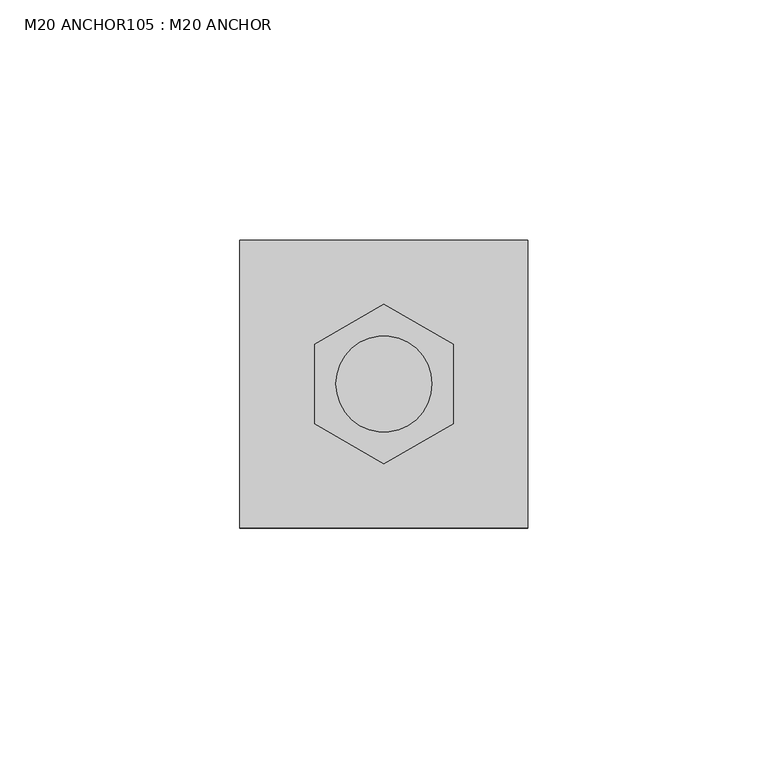
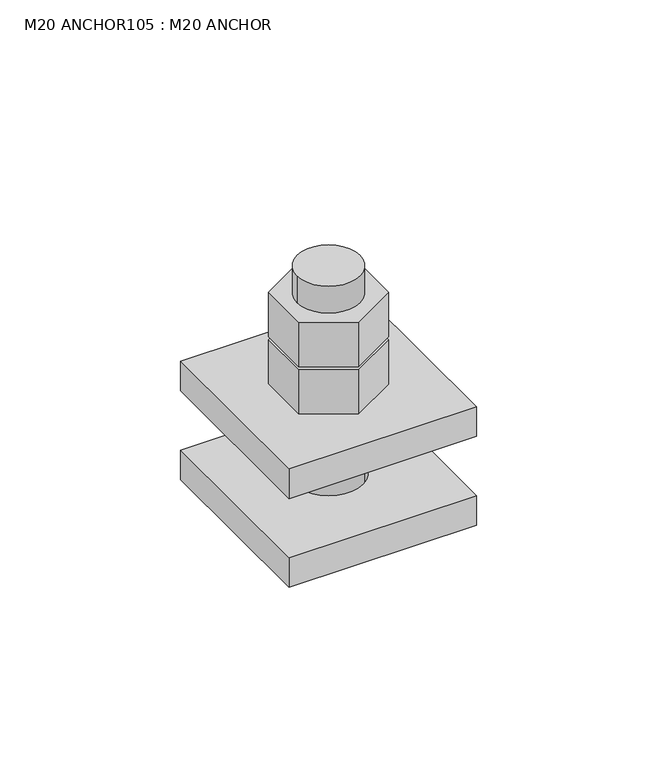
"""IFC4 building model written with IfcOpenShell, lengths in millimetres: fastener geometry, M20 ANCHOR105 : M20 ANCHOR."""

import ifcopenshell
import ifcopenshell.guid

model = None  # the IFC model being written
_history = None  # IfcOwnerHistory: only IFC2X3 demands one
_inside = {}  # id of a spatial element -> (the spatial element, [elements in it])
_under = {}  # id of a project, library or spatial element -> (it, [spatial elements below it])
_declared = {}  # id of a project -> (the project, [libraries it declares])
_typed = {}  # id of a type object -> (the type object, [elements of that type])
_made_of = {}  # id of a material, layer set ... -> (it, [elements and type objects made of it])


def new_model(schema):
    """Start an empty IFC model of exactly this schema.

    Asked for "IFC4X3", IfcOpenShell would pick the latest addendum, in which some entities
    have other attributes; the version numbers below select the first issue.
    IFC2X3 requires an IfcOwnerHistory on every rooted entity: one is made here for all.
    """
    global model, _history
    if schema == "IFC4X3":
        model = ifcopenshell.file(schema_version=(4, 3, 0, 0))
    else:
        model = ifcopenshell.file(schema=schema)
    _inside.clear()
    _under.clear()
    _declared.clear()
    _typed.clear()
    _made_of.clear()
    _history = None
    if model.schema == "IFC2X3":
        org = make("IfcOrganization", Name="unknown")
        user = make(
            "IfcPersonAndOrganization",
            ThePerson=make("IfcPerson", FamilyName="unknown"),
            TheOrganization=org,
        )
        app = make(
            "IfcApplication",
            ApplicationDeveloper=org,
            Version="unknown",
            ApplicationFullName="unknown",
            ApplicationIdentifier="unknown",
        )
        _history = make(
            "IfcOwnerHistory",
            OwningUser=user,
            OwningApplication=app,
            ChangeAction="ADDED",
            CreationDate=0,
        )
    return model


def make(cls, **values):
    """One entity of the class cls with the attributes given. An attribute that is None is left unset."""
    return model.create_entity(
        cls, **{name: value for name, value in values.items() if value is not None}
    )


def rooted(cls, **values):
    """An entity with a GlobalId (a new one), such as an element, a storey or a relation."""
    return make(cls, GlobalId=ifcopenshell.guid.new(), OwnerHistory=_history, **values)


def si_unit(unit_type, name, prefix=None):
    """IfcSIUnit, for example si_unit("LENGTHUNIT", "METRE", prefix="MILLI")."""
    return make("IfcSIUnit", UnitType=unit_type, Prefix=prefix, Name=name)


def assignment(units):
    """IfcUnitAssignment: the units of a project."""
    return None if units is None else make("IfcUnitAssignment", Units=units)


def point(xyz):
    """IfcCartesianPoint."""
    return None if xyz is None else make("IfcCartesianPoint", Coordinates=xyz)


def direction(xyz):
    """IfcDirection."""
    return None if xyz is None else make("IfcDirection", DirectionRatios=xyz)


def frame(location, z_axis=None, x_axis=None):
    """IfcAxis2Placement3D, a coordinate frame: its origin and axes. An axis left out is left unset."""
    return make(
        "IfcAxis2Placement3D",
        Location=point(location),
        Axis=direction(z_axis),
        RefDirection=direction(x_axis),
    )


def frame_2d(location, x_axis=None):
    """IfcAxis2Placement2D, a coordinate frame in the plane: its origin and x axis."""
    return make(
        "IfcAxis2Placement2D", Location=point(location), RefDirection=direction(x_axis)
    )


def origin():
    """The frame at (0, 0, 0) with its axes left unset."""
    return frame((0.0, 0.0, 0.0))


def place(relative_to, where):
    """IfcLocalPlacement: puts the frame where relative to a parent placement (None: the world)."""
    return make(
        "IfcLocalPlacement", PlacementRelTo=relative_to, RelativePlacement=where
    )


def context(
    kind, dimensions, precision=None, world=None, true_north=None, identifier=None
):
    """IfcGeometricRepresentationContext, for example the 3D "Model" context."""
    return make(
        "IfcGeometricRepresentationContext",
        ContextIdentifier=identifier,
        ContextType=kind,
        CoordinateSpaceDimension=dimensions,
        Precision=precision,
        WorldCoordinateSystem=world,
        TrueNorth=true_north,
    )


def project(units=None, contexts=None):
    """IfcProject with its units and contexts."""
    return rooted(
        "IfcProject",
        Name="project",
        RepresentationContexts=contexts,
        UnitsInContext=assignment(units),
    )


def spatial(cls, under=None, at=None, **own):
    """A site, building, storey or space (cls), placed at a placement, below another one or the project."""
    s = rooted(cls, ObjectPlacement=at, **own)
    if under is not None:
        _under.setdefault(under.id(), (under, []))[1].append(s)
    return s


def polyline(points):
    """IfcPolyline through the points."""
    return make("IfcPolyline", Points=[point(p) for p in points])


def circle_curve(where, radius):
    """IfcCircle in the frame where."""
    return make("IfcCircle", Position=where, Radius=radius)


def trimmed(basis, trim1, trim2, sense, master):
    """IfcTrimmedCurve: the piece of a basis curve between two trims."""
    return make(
        "IfcTrimmedCurve",
        BasisCurve=basis,
        Trim1=trim1,
        Trim2=trim2,
        SenseAgreement=sense,
        MasterRepresentation=master,
    )


def segment(curve, same_sense, transition):
    """IfcCompositeCurveSegment."""
    return make(
        "IfcCompositeCurveSegment",
        Transition=transition,
        SameSense=same_sense,
        ParentCurve=curve,
    )


def composite_curve(segments, self_intersect=None):
    """IfcCompositeCurve: segments joined end to end."""
    return make("IfcCompositeCurve", Segments=segments, SelfIntersect=self_intersect)


def outline(outer, holes=None, kind="AREA"):
    """IfcArbitraryClosedProfileDef: a profile drawn as a closed curve; with holes, ...WithVoids."""
    if holes is None:
        return make("IfcArbitraryClosedProfileDef", ProfileType=kind, OuterCurve=outer)
    return make(
        "IfcArbitraryProfileDefWithVoids",
        ProfileType=kind,
        OuterCurve=outer,
        InnerCurves=holes,
    )


def extrude(swept, where, along, depth):
    """IfcExtrudedAreaSolid: the profile swept, set in the frame where, extruded along a direction by depth."""
    return make(
        "IfcExtrudedAreaSolid",
        SweptArea=swept,
        Position=where,
        ExtrudedDirection=direction(along),
        Depth=depth,
    )


def shape(context_of_items, identifier, shape_type, items):
    """IfcShapeRepresentation: the items that make up one representation, for example the "Body"."""
    return make(
        "IfcShapeRepresentation",
        ContextOfItems=context_of_items,
        RepresentationIdentifier=identifier,
        RepresentationType=shape_type,
        Items=items,
    )


def source(mapping_origin, context_of_items, identifier, shape_type, items):
    """IfcRepresentationMap: a shape defined once, which mapped items show again and again."""
    return make(
        "IfcRepresentationMap",
        MappingOrigin=mapping_origin,
        MappedRepresentation=shape(context_of_items, identifier, shape_type, items),
    )


def transform(
    local_origin,
    x_axis=None,
    y_axis=None,
    z_axis=None,
    scale=None,
    scale2=None,
    scale3=None,
    uniform=True,
):
    """IfcCartesianTransformationOperator3D, or its non-uniform kind. x_axis, y_axis, z_axis: its Axis1, 2, 3."""
    if uniform:
        return make(
            "IfcCartesianTransformationOperator3D",
            Axis1=direction(x_axis),
            Axis2=direction(y_axis),
            LocalOrigin=point(local_origin),
            Scale=scale,
            Axis3=direction(z_axis),
        )
    return make(
        "IfcCartesianTransformationOperator3DnonUniform",
        Axis1=direction(x_axis),
        Axis2=direction(y_axis),
        LocalOrigin=point(local_origin),
        Scale=scale,
        Axis3=direction(z_axis),
        Scale2=scale2,
        Scale3=scale3,
    )


def mapped(mapping_source, mapping_target):
    """IfcMappedItem: shows the shape of a source again, moved by a transform."""
    return make(
        "IfcMappedItem", MappingSource=mapping_source, MappingTarget=mapping_target
    )


def made_of(thing, what):
    """Note that an element or type object is made of a material, layer set ...; save() writes the relation."""
    if what is not None:
        _made_of.setdefault(what.id(), (what, []))[1].append(thing)
    return thing


def element(
    cls,
    number,
    at=None,
    inside=None,
    cuts=None,
    type_object=None,
    material=None,
    context=None,
    identifier="Body",
    shape_type=None,
    held_by="IfcProductDefinitionShape",
    body=None,
    shapes=None,
    **own,
):
    """One element of the class cls, such as IfcWall. Its Tag is "e" and its number.

    at: its placement. inside: the storey or other place that contains it. cuts: it is an
    opening in that element (IfcRelVoidsElement). A single representation is given by context,
    identifier, shape_type and body (its items); several are given by shapes. held_by: the class
    of the entity that holds the representations. save() writes the other relations.
    """
    e = rooted(cls, Tag="e%d" % number, ObjectPlacement=at, **own)
    if body is not None:
        shapes = [shape(context, identifier, shape_type, body)]
    if shapes is not None:
        e.Representation = make(held_by, Representations=shapes)
    if inside is not None:
        _inside.setdefault(inside.id(), (inside, []))[1].append(e)
    if cuts is not None:
        rooted(
            "IfcRelVoidsElement", RelatingBuildingElement=cuts, RelatedOpeningElement=e
        )
    if type_object is not None:
        _typed.setdefault(type_object.id(), (type_object, []))[1].append(e)
    return made_of(e, material)


def aggregate(whole, parts):
    """IfcRelAggregates: a whole, such as a stair, and the parts it consists of."""
    return rooted("IfcRelAggregates", RelatingObject=whole, RelatedObjects=parts)


def save(model, path):
    """Write the relations noted so far, then the file.

    IfcRelAggregates (storeys below a building ...), IfcRelContainedInSpatialStructure (elements
    in a storey), IfcRelDefinesByType, IfcRelAssociatesMaterial and IfcRelDeclares: one each for
    every whole, place, type object, material and project.
    """
    for whole, parts in _under.values():
        aggregate(whole, parts)
    for where, things in _inside.values():
        rooted(
            "IfcRelContainedInSpatialStructure",
            RelatedElements=things,
            RelatingStructure=where,
        )
    for kind, things in _typed.values():
        rooted("IfcRelDefinesByType", RelatedObjects=things, RelatingType=kind)
    for what, things in _made_of.values():
        rooted("IfcRelAssociatesMaterial", RelatedObjects=things, RelatingMaterial=what)
    for by, libraries in _declared.values():
        rooted("IfcRelDeclares", RelatingContext=by, RelatedDefinitions=libraries)
    model.write(path)


def m20_anchor105_m20_anchor_da761a71(model_context):
    return source(origin(), model_context, "Body", "SweptSolid", [
        extrude(outline(polyline([(15008.0855968, 22545.0952779), (15022.4937158, 22553.4138093), (15036.9018348, 22545.0952779), (15036.9018348, 22528.4582151), (15022.4937158, 22520.1396837), (15008.0855968, 22528.4582151), (15008.0855968, 22545.0952779)]), holes=[composite_curve([segment(trimmed(circle_curve(frame_2d((15022.4937158, 22536.7767465)), 10.0), [point((15032.4937158, 22536.7767465))], [point((15012.4937158, 22536.7767465))], True, "CARTESIAN"), True, "CONTINUOUS"), segment(trimmed(circle_curve(frame_2d((15022.4937158, 22536.7767465)), 10.0), [point((15012.4937158, 22536.7767465))], [point((15032.4937158, 22536.7767465))], True, "CARTESIAN"), True, "CONTINUOUS")], self_intersect=False)]), frame((0.0, 0.0, 246.0), z_axis=(0.0, 0.0, 1.0), x_axis=(1.0, 0.0, 0.0)), (0.0, 0.0, 1.0), 15.0),
        extrude(outline(polyline([(15008.0855968, 22545.0952779), (15022.4937158, 22553.4138093), (15036.9018348, 22545.0952779), (15036.9018348, 22528.4582151), (15022.4937158, 22520.1396837), (15008.0855968, 22528.4582151), (15008.0855968, 22545.0952779)]), holes=[composite_curve([segment(trimmed(circle_curve(frame_2d((15022.4937158, 22536.7767465)), 10.0), [point((15032.4937158, 22536.7767465))], [point((15012.4937158, 22536.7767465))], True, "CARTESIAN"), True, "CONTINUOUS"), segment(trimmed(circle_curve(frame_2d((15022.4937158, 22536.7767465)), 10.0), [point((15012.4937158, 22536.7767465))], [point((15032.4937158, 22536.7767465))], True, "CARTESIAN"), True, "CONTINUOUS")], self_intersect=False)]), frame((0.0, 0.0, 230.0), z_axis=(0.0, 0.0, 1.0), x_axis=(1.0, 0.0, 0.0)), (0.0, 0.0, 1.0), 15.0),
        extrude(outline(composite_curve([segment(trimmed(circle_curve(frame_2d((15022.4937158, 22536.7767465)), 10.0), [point((15032.4937158, 22536.7767465))], [point((15012.4937158, 22536.7767465))], False, "CARTESIAN"), True, "CONTINUOUS"), segment(trimmed(circle_curve(frame_2d((15022.4937158, 22536.7767465)), 10.0), [point((15012.4937158, 22536.7767465))], [point((15032.4937158, 22536.7767465))], False, "CARTESIAN"), True, "CONTINUOUS")], self_intersect=False)), frame((0.0, 0.0, 190.0), z_axis=(0.0, 0.0, 1.0), x_axis=(1.0, 0.0, 0.0)), (0.0, 0.0, 1.0), 80.0),
        extrude(outline(polyline([(14992.4937158, 22566.7767465), (15052.4937158, 22566.7767465), (15052.4937158, 22506.7767465), (14992.4937158, 22506.7767465), (14992.4937158, 22566.7767465)]), holes=[composite_curve([segment(trimmed(circle_curve(frame_2d((15022.4937158, 22536.7767465)), 11.0), [point((15033.4937158, 22536.7767465))], [point((15011.4937158, 22536.7767465))], True, "CARTESIAN"), True, "CONTINUOUS"), segment(trimmed(circle_curve(frame_2d((15022.4937158, 22536.7767465)), 11.0), [point((15011.4937158, 22536.7767465))], [point((15033.4937158, 22536.7767465))], True, "CARTESIAN"), True, "CONTINUOUS")], self_intersect=False)]), frame((0.0, 0.0, 190.0), z_axis=(0.0, 0.0, 1.0), x_axis=(1.0, 0.0, 0.0)), (0.0, 0.0, 1.0), 10.0),
        extrude(outline(polyline([(14992.4937158, 22566.7767465), (15052.4937158, 22566.7767465), (15052.4937158, 22506.7767465), (14992.4937158, 22506.7767465), (14992.4937158, 22566.7767465)]), holes=[composite_curve([segment(trimmed(circle_curve(frame_2d((15022.4937158, 22536.7767465)), 11.0), [point((15033.4937158, 22536.7767465))], [point((15011.4937158, 22536.7767465))], True, "CARTESIAN"), True, "CONTINUOUS"), segment(trimmed(circle_curve(frame_2d((15022.4937158, 22536.7767465)), 11.0), [point((15011.4937158, 22536.7767465))], [point((15033.4937158, 22536.7767465))], True, "CARTESIAN"), True, "CONTINUOUS")], self_intersect=False)]), frame((0.0, 0.0, 220.0), z_axis=(0.0, 0.0, 1.0), x_axis=(1.0, 0.0, 0.0)), (0.0, 0.0, 1.0), 10.0),
    ])


if __name__ == "__main__":
    model = new_model("IFC4")
    model_context = context("Model", 3, world=origin())
    ifc_project = project(units=[si_unit("LENGTHUNIT", "METRE", prefix="MILLI")], contexts=[model_context])
    site = spatial("IfcSite", under=ifc_project)
    building = spatial("IfcBuilding", under=site)
    placement = place(None, origin())
    m20_anchor105_m20_anchor_shape = m20_anchor105_m20_anchor_da761a71(model_context)
    element("IfcFastener", 1, ObjectType="M20 ANCHOR105 : M20 ANCHOR", at=placement, inside=building, context=model_context, shape_type="MappedRepresentation", body=[
        mapped(m20_anchor105_m20_anchor_shape, transform((0.0, 0.0, 0.0), x_axis=(1.0, 0.0, 0.0), y_axis=(0.0, 1.0, 0.0), z_axis=(0.0, 0.0, 1.0))),
    ])
    save(model, "model.ifc")
